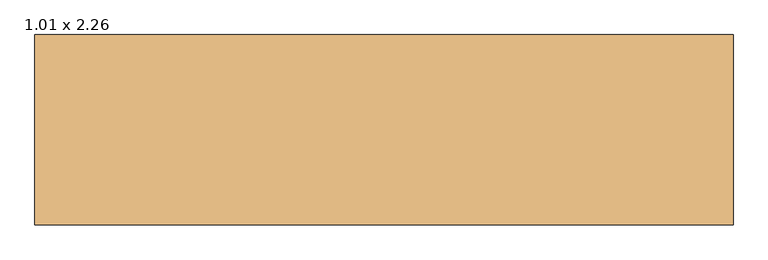
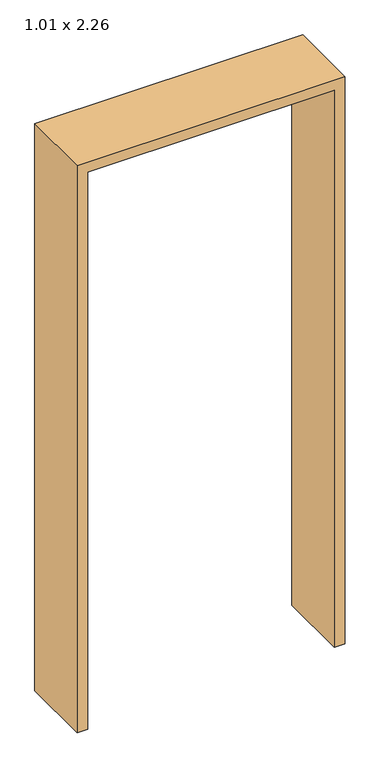
"""IFC4 building model written with IfcOpenShell, lengths in millimetres: door geometry, Durchfahrt - Blockzarge : 1.01 x 2.26."""

from ifc_helpers import new_model, si_unit, frame, origin, place, context, project, spatial, polyline, outline, extrude, source, transform, mapped, element, save


def door_1_01_x_2_26_265f3a24(model_context):
    return source(origin(), model_context, "Body", "SweptSolid", [
        extrude(outline(polyline([(2360.0, 505.0), (2360.0, -505.0), (100.0, -505.0), (100.0, -465.0), (2320.0, -465.0), (2320.0, 465.0), (100.0, 465.0), (100.0, 505.0), (2360.0, 505.0)])), frame((0.0, -123.0653859, 0.0), z_axis=(0.0, 1.0, 0.0), x_axis=(0.0, 0.0, 1.0)), (0.0, 0.0, 1.0), 275.0),
    ])


if __name__ == "__main__":
    model = new_model("IFC4")
    model_context = context("Model", 3, world=origin())
    ifc_project = project(units=[si_unit("LENGTHUNIT", "METRE", prefix="MILLI")], contexts=[model_context])
    site = spatial("IfcSite", under=ifc_project)
    building = spatial("IfcBuilding", under=site)
    placement = place(None, origin())
    door_1_01_x_2_26_shape = door_1_01_x_2_26_265f3a24(model_context)
    element("IfcDoor", 1, ObjectType="Durchfahrt - Blockzarge : 1.01 x 2.26", at=placement, inside=building, context=model_context, shape_type="MappedRepresentation", body=[
        mapped(door_1_01_x_2_26_shape, transform((0.0, 0.0, 0.0), x_axis=(1.0, 0.0, 0.0), y_axis=(0.0, 1.0, 0.0), z_axis=(0.0, 0.0, 1.0))),
    ])
    save(model, "model.ifc")

# Revit data of these elements
# Type "Durchfahrt - Blockzarge : 1.01 x 2.26"
#   Type Mark = "22"
#   Keynote = "16.03"
#   Rough Width = 1.010 m
#   Stärke Futter = 0.040 m
#   Rough Height [instance default] = 2.360 m
#   Height = 2.260 m
#   Fußbodenaufbau [instance default] = 0.100 m
#   Width = 1.010 m
#   Sichtbarkeit Sturzlinien [instance default] = yes
#   Rahmen/Pfosten = none
#   Function = (empty or 0)
#   Wall Closure = (empty or 0)
# Element 1 (IfcDoor, "Durchfahrt - Blockzarge : 1.01 x 2.26")
#   Materials on its faces: "Holz - Birke"
# Materials
#   "Holz - Birke": class "Holz", colour RGB 213 164 103, transparency 0, Cost = 0
